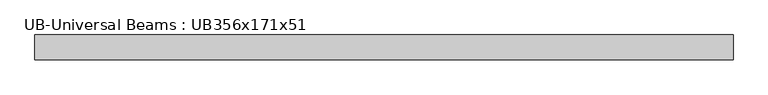
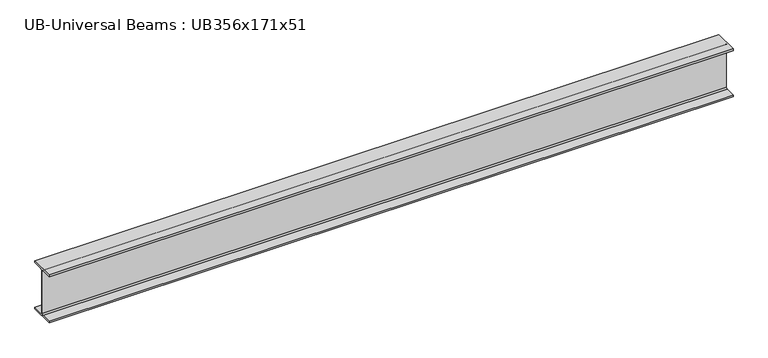
"""IFC4 building model written with IfcOpenShell, lengths in millimetres: beam geometry, UB-Universal Beams : UB356x171x51."""

from ifc_helpers import new_model, si_unit, point, frame, frame_2d, origin, place, context, project, spatial, polyline, circle_curve, trimmed, segment, composite_curve, outline, extrude, source, transform, mapped, element, save


def ub_universal_beams_ub356x171x51_7273abb1(model_context):
    return source(origin(), model_context, "Body", "SweptSolid", [
        extrude(outline(composite_curve([segment(polyline([(85.75, -166.0), (85.75, -177.5), (-85.75, -177.5), (-85.75, -166.0), (-13.9, -166.0)]), True, "CONTINUOUS"), segment(trimmed(circle_curve(frame_2d((-13.9, -155.8)), 10.2), [point((-13.9, -166.0))], [point((-3.7, -155.8))], True, "CARTESIAN"), True, "CONTINUOUS"), segment(polyline([(-3.7, -155.8), (-3.7, 155.8)]), True, "CONTINUOUS"), segment(trimmed(circle_curve(frame_2d((-13.9, 155.8)), 10.2), [point((-3.7, 155.8))], [point((-13.9, 166.0))], True, "CARTESIAN"), True, "CONTINUOUS"), segment(polyline([(-13.9, 166.0), (-85.75, 166.0), (-85.75, 177.5), (85.75, 177.5), (85.75, 166.0), (13.9, 166.0)]), True, "CONTINUOUS"), segment(trimmed(circle_curve(frame_2d((13.9, 155.8)), 10.2), [point((13.9, 166.0))], [point((3.7, 155.8))], True, "CARTESIAN"), True, "CONTINUOUS"), segment(polyline([(3.7, 155.8), (3.7, -155.8)]), True, "CONTINUOUS"), segment(trimmed(circle_curve(frame_2d((13.9, -155.8)), 10.2), [point((3.7, -155.8))], [point((13.9, -166.0))], True, "CARTESIAN"), True, "CONTINUOUS"), segment(polyline([(13.9, -166.0), (85.75, -166.0)]), True, "CONTINUOUS")], self_intersect=False)), frame((-2416.9, 0.0, 0.0), z_axis=(1.0, 0.0, 0.0), x_axis=(0.0, 1.0, 0.0)), (0.0, 0.0, 1.0), 4789.9),
    ])


if __name__ == "__main__":
    model = new_model("IFC4")
    model_context = context("Model", 3, world=origin())
    ifc_project = project(units=[si_unit("LENGTHUNIT", "METRE", prefix="MILLI")], contexts=[model_context])
    site = spatial("IfcSite", under=ifc_project)
    building = spatial("IfcBuilding", under=site)
    placement = place(None, origin())
    ub_universal_beams_ub356x171x51_shape = ub_universal_beams_ub356x171x51_7273abb1(model_context)
    element("IfcBeam", 1, ObjectType="UB-Universal Beams : UB356x171x51", at=placement, inside=building, context=model_context, shape_type="MappedRepresentation", body=[
        mapped(ub_universal_beams_ub356x171x51_shape, transform((0.0, 0.0, 0.0), x_axis=(1.0, 0.0, 0.0), y_axis=(0.0, 1.0, 0.0), z_axis=(0.0, 0.0, 1.0))),
    ])
    save(model, "model.ifc")

# Revit data of these elements
# Type "UB-Universal Beams : UB356x171x51"
#   Section Name Key = "UB356X171X51"
#   Width = 17.15 cm
#   Web Thickness = 0.74 cm
#   Web Fillet = 1.02 cm
#   Warping Constant = 286000.0 cm⁶
#   Torsional Moment of Inertia = 23.80 cm⁴
#   Section Area = 64.9 cm²
#   Plastic Modulus weak axis = 174.0 cm³
#   Plastic Modulus strong axis = 896.0 cm³
#   Nominal Weight = 50.9998 kgf/m
#   Moment of Inertia weak axis = 968.00 cm⁴
#   Moment of Inertia strong axis = 14136.00 cm⁴
#   Height = 35.5 cm
#   Flange Thickness = 1.15 cm
#   Elastic Modulus weak axis = 113.0 cm³
#   Elastic Modulus strong axis = 796.0 cm³
#   Centroid Vertical = 17.75 cm
#   Centroid Horizontal = 8.575 cm
#   Bolt Spacing = 9.0 cm
#   Length [instance default] = 1500 mm
#   Structural Material [instance default] = Metal - Steel 43-275
#   Type Comments = ""
#   Assembly Code = ""
# Element 1 (IfcBeam, "UB-Universal Beams : UB356x171x51")
#   Materials on its faces: "Metal - Steel 43-275"
# Materials
#   "Metal - Steel 43-275": class "Metal", colour RGB 247 247 247, transparency 0, Cost = 0
